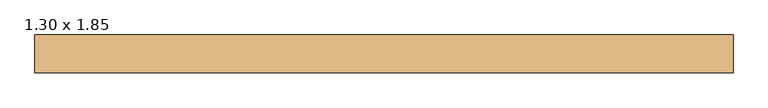
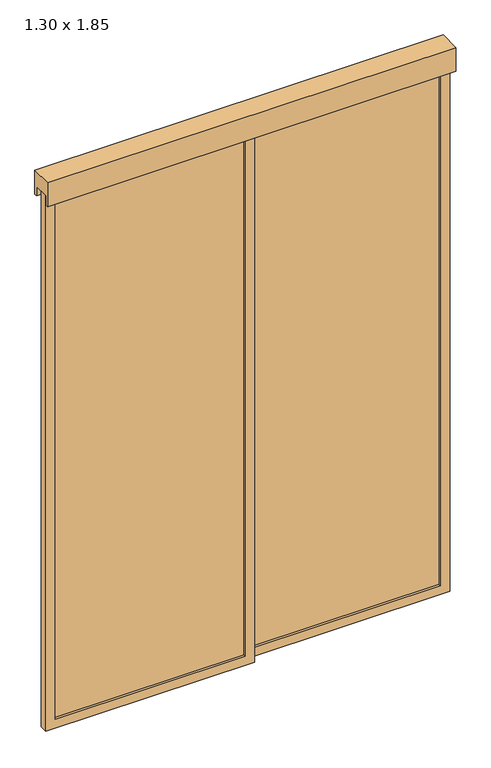
"""IFC4 building model written with IfcOpenShell, lengths in millimetres: door geometry, CC_BOX VIDRO RETO : 1.30 x 1.85."""

import ifcopenshell
import ifcopenshell.guid

model = None  # the IFC model being written
_history = None  # IfcOwnerHistory: only IFC2X3 demands one
_inside = {}  # id of a spatial element -> (the spatial element, [elements in it])
_under = {}  # id of a project, library or spatial element -> (it, [spatial elements below it])
_declared = {}  # id of a project -> (the project, [libraries it declares])
_typed = {}  # id of a type object -> (the type object, [elements of that type])
_made_of = {}  # id of a material, layer set ... -> (it, [elements and type objects made of it])


def new_model(schema):
    """Start an empty IFC model of exactly this schema.

    Asked for "IFC4X3", IfcOpenShell would pick the latest addendum, in which some entities
    have other attributes; the version numbers below select the first issue.
    IFC2X3 requires an IfcOwnerHistory on every rooted entity: one is made here for all.
    """
    global model, _history
    if schema == "IFC4X3":
        model = ifcopenshell.file(schema_version=(4, 3, 0, 0))
    else:
        model = ifcopenshell.file(schema=schema)
    _inside.clear()
    _under.clear()
    _declared.clear()
    _typed.clear()
    _made_of.clear()
    _history = None
    if model.schema == "IFC2X3":
        org = make("IfcOrganization", Name="unknown")
        user = make(
            "IfcPersonAndOrganization",
            ThePerson=make("IfcPerson", FamilyName="unknown"),
            TheOrganization=org,
        )
        app = make(
            "IfcApplication",
            ApplicationDeveloper=org,
            Version="unknown",
            ApplicationFullName="unknown",
            ApplicationIdentifier="unknown",
        )
        _history = make(
            "IfcOwnerHistory",
            OwningUser=user,
            OwningApplication=app,
            ChangeAction="ADDED",
            CreationDate=0,
        )
    return model


def make(cls, **values):
    """One entity of the class cls with the attributes given. An attribute that is None is left unset."""
    return model.create_entity(
        cls, **{name: value for name, value in values.items() if value is not None}
    )


def rooted(cls, **values):
    """An entity with a GlobalId (a new one), such as an element, a storey or a relation."""
    return make(cls, GlobalId=ifcopenshell.guid.new(), OwnerHistory=_history, **values)


def si_unit(unit_type, name, prefix=None):
    """IfcSIUnit, for example si_unit("LENGTHUNIT", "METRE", prefix="MILLI")."""
    return make("IfcSIUnit", UnitType=unit_type, Prefix=prefix, Name=name)


def assignment(units):
    """IfcUnitAssignment: the units of a project."""
    return None if units is None else make("IfcUnitAssignment", Units=units)


def point(xyz):
    """IfcCartesianPoint."""
    return None if xyz is None else make("IfcCartesianPoint", Coordinates=xyz)


def direction(xyz):
    """IfcDirection."""
    return None if xyz is None else make("IfcDirection", DirectionRatios=xyz)


def frame(location, z_axis=None, x_axis=None):
    """IfcAxis2Placement3D, a coordinate frame: its origin and axes. An axis left out is left unset."""
    return make(
        "IfcAxis2Placement3D",
        Location=point(location),
        Axis=direction(z_axis),
        RefDirection=direction(x_axis),
    )


def origin():
    """The frame at (0, 0, 0) with its axes left unset."""
    return frame((0.0, 0.0, 0.0))


def place(relative_to, where):
    """IfcLocalPlacement: puts the frame where relative to a parent placement (None: the world)."""
    return make(
        "IfcLocalPlacement", PlacementRelTo=relative_to, RelativePlacement=where
    )


def context(
    kind, dimensions, precision=None, world=None, true_north=None, identifier=None
):
    """IfcGeometricRepresentationContext, for example the 3D "Model" context."""
    return make(
        "IfcGeometricRepresentationContext",
        ContextIdentifier=identifier,
        ContextType=kind,
        CoordinateSpaceDimension=dimensions,
        Precision=precision,
        WorldCoordinateSystem=world,
        TrueNorth=true_north,
    )


def project(units=None, contexts=None):
    """IfcProject with its units and contexts."""
    return rooted(
        "IfcProject",
        Name="project",
        RepresentationContexts=contexts,
        UnitsInContext=assignment(units),
    )


def spatial(cls, under=None, at=None, **own):
    """A site, building, storey or space (cls), placed at a placement, below another one or the project."""
    s = rooted(cls, ObjectPlacement=at, **own)
    if under is not None:
        _under.setdefault(under.id(), (under, []))[1].append(s)
    return s


def polyline(points):
    """IfcPolyline through the points."""
    return make("IfcPolyline", Points=[point(p) for p in points])


def outline(outer, holes=None, kind="AREA"):
    """IfcArbitraryClosedProfileDef: a profile drawn as a closed curve; with holes, ...WithVoids."""
    if holes is None:
        return make("IfcArbitraryClosedProfileDef", ProfileType=kind, OuterCurve=outer)
    return make(
        "IfcArbitraryProfileDefWithVoids",
        ProfileType=kind,
        OuterCurve=outer,
        InnerCurves=holes,
    )


def extrude(swept, where, along, depth):
    """IfcExtrudedAreaSolid: the profile swept, set in the frame where, extruded along a direction by depth."""
    return make(
        "IfcExtrudedAreaSolid",
        SweptArea=swept,
        Position=where,
        ExtrudedDirection=direction(along),
        Depth=depth,
    )


def shape(context_of_items, identifier, shape_type, items):
    """IfcShapeRepresentation: the items that make up one representation, for example the "Body"."""
    return make(
        "IfcShapeRepresentation",
        ContextOfItems=context_of_items,
        RepresentationIdentifier=identifier,
        RepresentationType=shape_type,
        Items=items,
    )


def source(mapping_origin, context_of_items, identifier, shape_type, items):
    """IfcRepresentationMap: a shape defined once, which mapped items show again and again."""
    return make(
        "IfcRepresentationMap",
        MappingOrigin=mapping_origin,
        MappedRepresentation=shape(context_of_items, identifier, shape_type, items),
    )


def transform(
    local_origin,
    x_axis=None,
    y_axis=None,
    z_axis=None,
    scale=None,
    scale2=None,
    scale3=None,
    uniform=True,
):
    """IfcCartesianTransformationOperator3D, or its non-uniform kind. x_axis, y_axis, z_axis: its Axis1, 2, 3."""
    if uniform:
        return make(
            "IfcCartesianTransformationOperator3D",
            Axis1=direction(x_axis),
            Axis2=direction(y_axis),
            LocalOrigin=point(local_origin),
            Scale=scale,
            Axis3=direction(z_axis),
        )
    return make(
        "IfcCartesianTransformationOperator3DnonUniform",
        Axis1=direction(x_axis),
        Axis2=direction(y_axis),
        LocalOrigin=point(local_origin),
        Scale=scale,
        Axis3=direction(z_axis),
        Scale2=scale2,
        Scale3=scale3,
    )


def mapped(mapping_source, mapping_target):
    """IfcMappedItem: shows the shape of a source again, moved by a transform."""
    return make(
        "IfcMappedItem", MappingSource=mapping_source, MappingTarget=mapping_target
    )


def made_of(thing, what):
    """Note that an element or type object is made of a material, layer set ...; save() writes the relation."""
    if what is not None:
        _made_of.setdefault(what.id(), (what, []))[1].append(thing)
    return thing


def element(
    cls,
    number,
    at=None,
    inside=None,
    cuts=None,
    type_object=None,
    material=None,
    context=None,
    identifier="Body",
    shape_type=None,
    held_by="IfcProductDefinitionShape",
    body=None,
    shapes=None,
    **own,
):
    """One element of the class cls, such as IfcWall. Its Tag is "e" and its number.

    at: its placement. inside: the storey or other place that contains it. cuts: it is an
    opening in that element (IfcRelVoidsElement). A single representation is given by context,
    identifier, shape_type and body (its items); several are given by shapes. held_by: the class
    of the entity that holds the representations. save() writes the other relations.
    """
    e = rooted(cls, Tag="e%d" % number, ObjectPlacement=at, **own)
    if body is not None:
        shapes = [shape(context, identifier, shape_type, body)]
    if shapes is not None:
        e.Representation = make(held_by, Representations=shapes)
    if inside is not None:
        _inside.setdefault(inside.id(), (inside, []))[1].append(e)
    if cuts is not None:
        rooted(
            "IfcRelVoidsElement", RelatingBuildingElement=cuts, RelatedOpeningElement=e
        )
    if type_object is not None:
        _typed.setdefault(type_object.id(), (type_object, []))[1].append(e)
    return made_of(e, material)


def aggregate(whole, parts):
    """IfcRelAggregates: a whole, such as a stair, and the parts it consists of."""
    return rooted("IfcRelAggregates", RelatingObject=whole, RelatedObjects=parts)


def save(model, path):
    """Write the relations noted so far, then the file.

    IfcRelAggregates (storeys below a building ...), IfcRelContainedInSpatialStructure (elements
    in a storey), IfcRelDefinesByType, IfcRelAssociatesMaterial and IfcRelDeclares: one each for
    every whole, place, type object, material and project.
    """
    for whole, parts in _under.values():
        aggregate(whole, parts)
    for where, things in _inside.values():
        rooted(
            "IfcRelContainedInSpatialStructure",
            RelatedElements=things,
            RelatingStructure=where,
        )
    for kind, things in _typed.values():
        rooted("IfcRelDefinesByType", RelatedObjects=things, RelatingType=kind)
    for what, things in _made_of.values():
        rooted("IfcRelAssociatesMaterial", RelatedObjects=things, RelatingMaterial=what)
    for by, libraries in _declared.values():
        rooted("IfcRelDeclares", RelatingContext=by, RelatedDefinitions=libraries)
    model.write(path)


def door_1_30_x_1_85_06d559d3(model_context):
    return source(origin(), model_context, "Body", "SweptSolid", [
        extrude(outline(polyline([(620.0, 7.5), (15.0, 7.5), (15.0, 17.5), (620.0, 17.5), (620.0, 7.5)])), frame((0.0, 0.0, 30.0), z_axis=(0.0, 0.0, 1.0), x_axis=(1.0, 0.0, 0.0)), (0.0, 0.0, 1.0), 1740.0),
        extrude(outline(polyline([(1800.0, 650.0), (1800.0, -15.0), (0.0, -15.0), (0.0, 650.0), (1800.0, 650.0)]), holes=[polyline([(1770.0, 620.0), (30.0, 620.0), (30.0, 15.0), (1770.0, 15.0), (1770.0, 620.0)])]), frame((0.0, 0.0, 0.0), z_axis=(0.0, 1.0, 0.0), x_axis=(0.0, 0.0, 1.0)), (0.0, 0.0, 1.0), 25.0),
        extrude(outline(polyline([(-15.0, -17.5), (-620.0, -17.5), (-620.0, -7.5), (-15.0, -7.5), (-15.0, -17.5)])), frame((0.0, 0.0, 30.0), z_axis=(0.0, 0.0, 1.0), x_axis=(1.0, 0.0, 0.0)), (0.0, 0.0, 1.0), 1740.0),
        extrude(outline(polyline([(1800.0, 15.0), (1800.0, -650.0), (0.0, -650.0), (0.0, 15.0), (1800.0, 15.0)]), holes=[polyline([(1770.0, -15.0), (30.0, -15.0), (30.0, -620.0), (1770.0, -620.0), (1770.0, -15.0)])]), frame((0.0, -25.0, 0.0), z_axis=(0.0, 1.0, 0.0), x_axis=(0.0, 0.0, 1.0)), (0.0, 0.0, 1.0), 25.0),
        extrude(outline(polyline([(-25.0, 1800.0), (-25.0, 1770.0), (-35.0, 1770.0), (-35.0, 1850.0), (35.0, 1850.0), (35.0, 1770.0), (25.0, 1770.0), (25.0, 1800.0), (-25.0, 1800.0)])), frame((-650.0, 0.0, 0.0), z_axis=(1.0, 0.0, 0.0), x_axis=(0.0, 1.0, 0.0)), (0.0, 0.0, 1.0), 1300.0),
    ])


if __name__ == "__main__":
    model = new_model("IFC4")
    model_context = context("Model", 3, world=origin())
    ifc_project = project(units=[si_unit("LENGTHUNIT", "METRE", prefix="MILLI")], contexts=[model_context])
    site = spatial("IfcSite", under=ifc_project)
    building = spatial("IfcBuilding", under=site)
    placement = place(None, origin())
    door_1_30_x_1_85_shape = door_1_30_x_1_85_06d559d3(model_context)
    element("IfcDoor", 1, ObjectType="CC_BOX VIDRO RETO : 1.30 x 1.85", at=placement, inside=building, context=model_context, shape_type="MappedRepresentation", body=[
        mapped(door_1_30_x_1_85_shape, transform((0.0, 0.0, 0.0), x_axis=(1.0, 0.0, 0.0), y_axis=(0.0, 1.0, 0.0), z_axis=(0.0, 0.0, 1.0))),
    ])
    save(model, "model.ifc")

# Revit data of these elements
# Type "CC_BOX VIDRO RETO : 1.30 x 1.85"
#   Type Mark = "BOX"
#   Site = "www.construir.arq.br"
#   Empresa = "Cursos Construir"
#   Criado Por = "Roberto Netto"
#   Analytic Construction = "<Nenhum>"
#   Atualizado por = "Rudemberg Eloi"
#   Rough Width = 1.30 m
#   Largura Moldura [instance default] = 0.03 m
#   Largura Folha [instance default] = 0.665 m
#   Width = 1.30 m
#   Espessura Vidro [instance default] = 0.01 m
#   Espessura Folha [instance default] = 0.025 m
#   Thickness = 0.05 m
#   Rough Height = 1.85 m
#   Altura Folha [instance default] = 1.80 m
#   Height = 1.85 m
#   ----FOLHA---- [instance default] = 0.00 m
#   Material Vidro = .VIDRO
#   Material Trilho = .ALUMÍNIO COM PINTURA ELETROSTÁTICA BRANCA
#   Material Moldura = .ALUMÍNIO COM PINTURA ELETROSTÁTICA BRANCA
#   Function = (empty or 0)
#   Description = (empty or 0)
# Element 1 (IfcDoor, "CC_BOX VIDRO RETO : 1.30 x 1.85")
#   Materials on its faces: ".ALUMÍNIO COM PINTURA ELETROSTÁTICA BRANCA", ".VIDRO"
# Materials
#   ".VIDRO": class "Genérico", colour RGB 198 236 255, transparency 0.95, Cost = 0
#   ".ALUMÍNIO COM PINTURA ELETROSTÁTICA BRANCA": class "CC_METAIS", colour RGB 241 241 241, transparency 0, Cost = 0
